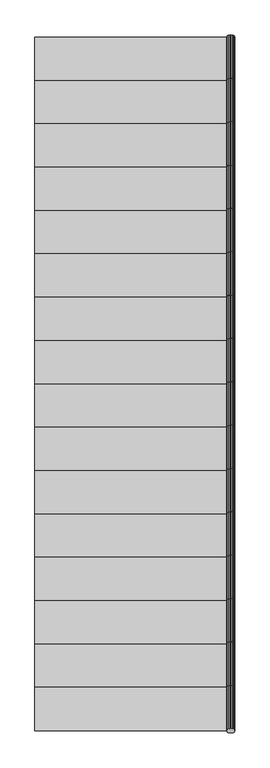
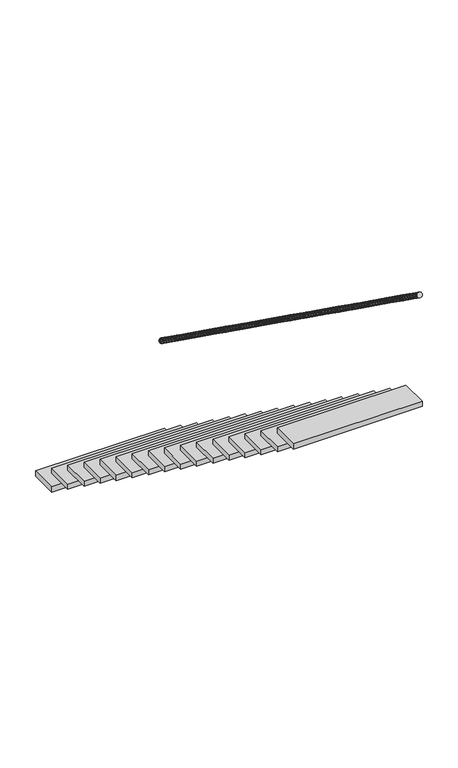
"""IFC4 building model written with IfcOpenShell, lengths in millimetres: stair geometry, 0_3d."""

from ifc_helpers import new_model, si_unit, frame, origin, origin_with_axes, place, context, project, spatial, polyline, outline, extrude, source, transform, mapped, element, save


def stair_45912ed6(model_context):
    return source(origin(), model_context, "Body", "SweptSolid", [
        extrude(outline(polyline([(1.2235871, -7.1914682), (0.0, 0.0), (1.2235871, 7.1914683), (4.7745751, 13.6789855), (10.3053687, 18.8275083), (17.2745751, 22.1330636), (25.0, 23.2720802), (32.7254249, 22.1330636), (39.6946313, 18.8275083), (45.2254249, 13.6789855), (48.7764129, 7.1914683), (50.0, 0.0), (48.7764129, -7.1914682), (45.2254249, -13.6789855), (39.6946313, -18.8275083), (32.7254249, -22.1330635), (25.0, -23.2720801), (17.2745751, -22.1330635), (10.3053687, -18.8275083), (4.7745751, -13.6789855), (1.2235871, -7.1914682)])), frame((1150.0, 3653.5347238, 1292.7647059), z_axis=(0.0, -0.8134846854822023, 0.5815863362269806), x_axis=(1.0, 0.0, 0.0)), (0.0, 0.0, 1.0), 319.6126548),
        extrude(outline(polyline([(1.2235871, -7.1914682), (0.0, 0.0), (1.2235871, 7.1914683), (4.7745751, 13.6789855), (10.3053687, 18.8275083), (17.2745751, 22.1330636), (25.0, 23.2720802), (32.7254249, 22.1330636), (39.6946313, 18.8275083), (45.2254249, 13.6789855), (48.7764129, 7.1914683), (50.0, 0.0), (48.7764129, -7.1914682), (45.2254249, -13.6789855), (39.6946313, -18.8275083), (32.7254249, -22.1330635), (25.0, -23.2720801), (17.2745751, -22.1330635), (10.3053687, -18.8275083), (4.7745751, -13.6789855), (1.2235871, -7.1914682)])), frame((1150.0, 4173.5347238, 921.0), z_axis=(0.0, -0.8134846854822141, 0.5815863362269641), x_axis=(1.0, 0.0, 0.0)), (0.0, 0.0, 1.0), 319.6126548),
        extrude(outline(polyline([(1.2235871, -7.1914682), (0.0, 0.0), (1.2235871, 7.1914683), (4.7745751, 13.6789855), (10.3053687, 18.8275083), (17.2745751, 22.1330636), (25.0, 23.2720802), (32.7254249, 22.1330636), (39.6946313, 18.8275083), (45.2254249, 13.6789855), (48.7764129, 7.1914683), (50.0, 0.0), (48.7764129, -7.1914682), (45.2254249, -13.6789855), (39.6946313, -18.8275083), (32.7254249, -22.1330635), (25.0, -23.2720801), (17.2745751, -22.1330635), (10.3053687, -18.8275083), (4.7745751, -13.6789855), (1.2235871, -7.1914682)])), frame((1150.0, 1833.5347238, 2593.9411765), z_axis=(0.0, -0.8134846854822316, 0.5815863362269396), x_axis=(1.0, 0.0, 0.0)), (0.0, 0.0, 1.0), 319.6126548),
        extrude(outline(polyline([(1.2235871, -7.1914682), (0.0, 0.0), (1.2235871, 7.1914683), (4.7745751, 13.6789855), (10.3053687, 18.8275083), (17.2745751, 22.1330636), (25.0, 23.2720802), (32.7254249, 22.1330636), (39.6946313, 18.8275083), (45.2254249, 13.6789855), (48.7764129, 7.1914683), (50.0, 0.0), (48.7764129, -7.1914682), (45.2254249, -13.6789855), (39.6946313, -18.8275083), (32.7254249, -22.1330635), (25.0, -23.2720801), (17.2745751, -22.1330635), (10.3053687, -18.8275083), (4.7745751, -13.6789855), (1.2235871, -7.1914682)])), frame((1150.0, 533.5347238, 3523.3529412), z_axis=(0.0, -0.8134846854822048, 0.581586336226977), x_axis=(1.0, 0.0, 0.0)), (0.0, 0.0, 1.0), 319.6126548),
        extrude(outline(polyline([(1.2235871, -7.1914682), (0.0, 0.0), (1.2235871, 7.1914683), (4.7745751, 13.6789855), (10.3053687, 18.8275083), (17.2745751, 22.1330636), (25.0, 23.2720802), (32.7254249, 22.1330636), (39.6946313, 18.8275083), (45.2254249, 13.6789855), (48.7764129, 7.1914683), (50.0, 0.0), (48.7764129, -7.1914682), (45.2254249, -13.6789855), (39.6946313, -18.8275083), (32.7254249, -22.1330635), (25.0, -23.2720801), (17.2745751, -22.1330635), (10.3053687, -18.8275083), (4.7745751, -13.6789855), (1.2235871, -7.1914682)])), frame((1150.0, 1053.5347238, 3151.5882353), z_axis=(0.0, -0.8134846854821998, 0.5815863362269841), x_axis=(1.0, 0.0, 0.0)), (0.0, 0.0, 1.0), 319.6126548),
        extrude(outline(polyline([(1.2235871, -7.1914682), (0.0, 0.0), (1.2235871, 7.1914683), (4.7745751, 13.6789855), (10.3053687, 18.8275083), (17.2745751, 22.1330636), (25.0, 23.2720802), (32.7254249, 22.1330636), (39.6946313, 18.8275083), (45.2254249, 13.6789855), (48.7764129, 7.1914683), (50.0, 0.0), (48.7764129, -7.1914682), (45.2254249, -13.6789855), (39.6946313, -18.8275083), (32.7254249, -22.1330635), (25.0, -23.2720801), (17.2745751, -22.1330635), (10.3053687, -18.8275083), (4.7745751, -13.6789855), (1.2235871, -7.1914682)])), frame((1150.0, 1573.5347238, 2779.8235294), z_axis=(0.0, -0.8134846854822146, 0.5815863362269632), x_axis=(1.0, 0.0, 0.0)), (0.0, 0.0, 1.0), 319.6126548),
        extrude(outline(polyline([(1200.0, 4173.5347238), (1200.0, 3913.5347238), (0.0, 3913.5347238), (0.0, 4173.5347238), (1200.0, 4173.5347238)])), origin_with_axes(), (0.0, 0.0, 1.0), 50.0),
        extrude(outline(polyline([(1.2235871, -7.1914682), (0.0, 0.0), (1.2235871, 7.1914683), (4.7745751, 13.6789856), (10.3053687, 18.8275083), (17.2745751, 22.1330636), (25.0, 23.2720803), (32.7254249, 22.1330636), (39.6946313, 18.8275083), (45.2254249, 13.6789856), (48.7764129, 7.1914683), (50.0, 0.0), (48.7764129, -7.1914682), (45.2254249, -13.6789855), (39.6946313, -18.8275083), (32.7254249, -22.1330635), (25.0, -23.2720801), (17.2745751, -22.1330635), (10.3053687, -18.8275083), (4.7745751, -13.6789855), (1.2235871, -7.1914682)])), frame((1150.0, 793.5347238, 3337.4705882), z_axis=(0.0, -0.8134846854821957, 0.5815863362269899), x_axis=(1.0, 0.0, 0.0)), (0.0, 0.0, 1.0), 319.6126548),
        extrude(outline(polyline([(1200.0, 2353.5347238), (1200.0, 2093.5347238), (0.0, 2093.5347238), (0.0, 2353.5347238), (1200.0, 2353.5347238)])), frame((0.0, 0.0, 1301.1764706), z_axis=(0.0, 0.0, 1.0), x_axis=(1.0, 0.0, 0.0)), (0.0, 0.0, 1.0), 50.0),
        extrude(outline(polyline([(1200.0, 3133.5347238), (1200.0, 2873.5347238), (0.0, 2873.5347238), (0.0, 3133.5347238), (1200.0, 3133.5347238)])), frame((0.0, 0.0, 743.5294118), z_axis=(0.0, 0.0, 1.0), x_axis=(1.0, 0.0, 0.0)), (0.0, 0.0, 1.0), 50.0),
        extrude(outline(polyline([(1.2235871, -7.1914682), (0.0, 0.0), (1.2235871, 7.1914683), (4.7745751, 13.6789855), (10.3053687, 18.8275083), (17.2745751, 22.1330636), (25.0, 23.2720802), (32.7254249, 22.1330636), (39.6946313, 18.8275083), (45.2254249, 13.6789855), (48.7764129, 7.1914683), (50.0, 0.0), (48.7764129, -7.1914682), (45.2254249, -13.6789855), (39.6946313, -18.8275083), (32.7254249, -22.1330635), (25.0, -23.2720801), (17.2745751, -22.1330635), (10.3053687, -18.8275083), (4.7745751, -13.6789855), (1.2235871, -7.1914682)])), frame((1150.0, 2353.5347238, 2222.1764706), z_axis=(0.0, -0.8134846854822106, 0.5815863362269689), x_axis=(1.0, 0.0, 0.0)), (0.0, 0.0, 1.0), 319.6126548),
        extrude(outline(polyline([(1.2235871, -7.1914682), (0.0, 0.0), (1.2235871, 7.1914683), (4.7745751, 13.6789855), (10.3053687, 18.8275083), (17.2745751, 22.1330636), (25.0, 23.2720802), (32.7254249, 22.1330636), (39.6946313, 18.8275083), (45.2254249, 13.6789855), (48.7764129, 7.1914683), (50.0, 0.0), (48.7764129, -7.1914682), (45.2254249, -13.6789855), (39.6946313, -18.8275083), (32.7254249, -22.1330635), (25.0, -23.2720801), (17.2745751, -22.1330635), (10.3053687, -18.8275083), (4.7745751, -13.6789855), (1.2235871, -7.1914682)])), frame((1150.0, 273.5347238, 3709.2352941), z_axis=(0.0, -0.8134846854821822, 0.5815863362270085), x_axis=(1.0, 0.0, 0.0)), (0.0, 0.0, 1.0), 319.6126548),
        extrude(outline(polyline([(1200.0, 1313.5347238), (1200.0, 1053.5347238), (0.0, 1053.5347238), (0.0, 1313.5347238), (1200.0, 1313.5347238)])), frame((0.0, 0.0, 2044.7058824), z_axis=(0.0, 0.0, 1.0), x_axis=(1.0, 0.0, 0.0)), (0.0, 0.0, 1.0), 50.0),
        extrude(outline(polyline([(1200.0, 3913.5347238), (1200.0, 3653.5347238), (0.0, 3653.5347238), (0.0, 3913.5347238), (1200.0, 3913.5347238)])), frame((0.0, 0.0, 185.8823529), z_axis=(0.0, 0.0, 1.0), x_axis=(1.0, 0.0, 0.0)), (0.0, 0.0, 1.0), 50.0),
        extrude(outline(polyline([(1200.0, 533.5347238), (1200.0, 273.5347238), (0.0, 273.5347238), (0.0, 533.5347238), (1200.0, 533.5347238)])), frame((0.0, 0.0, 2602.3529412), z_axis=(0.0, 0.0, 1.0), x_axis=(1.0, 0.0, 0.0)), (0.0, 0.0, 1.0), 50.0),
        extrude(outline(polyline([(1200.0, 2093.5347238), (1200.0, 1833.5347238), (0.0, 1833.5347238), (0.0, 2093.5347238), (1200.0, 2093.5347238)])), frame((0.0, 0.0, 1487.0588235), z_axis=(0.0, 0.0, 1.0), x_axis=(1.0, 0.0, 0.0)), (0.0, 0.0, 1.0), 50.0),
        extrude(outline(polyline([(1200.0, 1053.5347238), (1200.0, 793.5347238), (0.0, 793.5347238), (0.0, 1053.5347238), (1200.0, 1053.5347238)])), frame((0.0, 0.0, 2230.5882353), z_axis=(0.0, 0.0, 1.0), x_axis=(1.0, 0.0, 0.0)), (0.0, 0.0, 1.0), 50.0),
        extrude(outline(polyline([(1200.0, 3393.5347238), (1200.0, 3133.5347238), (0.0, 3133.5347238), (0.0, 3393.5347238), (1200.0, 3393.5347238)])), frame((0.0, 0.0, 557.6470588), z_axis=(0.0, 0.0, 1.0), x_axis=(1.0, 0.0, 0.0)), (0.0, 0.0, 1.0), 50.0),
        extrude(outline(polyline([(1.2235871, -7.1914682), (0.0, 0.0), (1.2235871, 7.1914683), (4.7745751, 13.6789855), (10.3053687, 18.8275083), (17.2745751, 22.1330636), (25.0, 23.2720802), (32.7254249, 22.1330636), (39.6946313, 18.8275083), (45.2254249, 13.6789855), (48.7764129, 7.1914683), (50.0, 0.0), (48.7764129, -7.1914682), (45.2254249, -13.6789855), (39.6946313, -18.8275083), (32.7254249, -22.1330635), (25.0, -23.2720801), (17.2745751, -22.1330635), (10.3053687, -18.8275083), (4.7745751, -13.6789855), (1.2235871, -7.1914682)])), frame((1150.0, 2873.5347238, 1850.4117647), z_axis=(0.0, -0.813484685482208, 0.5815863362269725), x_axis=(1.0, 0.0, 0.0)), (0.0, 0.0, 1.0), 319.6126548),
        extrude(outline(polyline([(1200.0, 793.5347238), (1200.0, 533.5347238), (0.0, 533.5347238), (0.0, 793.5347238), (1200.0, 793.5347238)])), frame((0.0, 0.0, 2416.4705882), z_axis=(0.0, 0.0, 1.0), x_axis=(1.0, 0.0, 0.0)), (0.0, 0.0, 1.0), 50.0),
        extrude(outline(polyline([(1200.0, 273.5347238), (1200.0, 13.5347238), (0.0, 13.5347238), (0.0, 273.5347238), (1200.0, 273.5347238)])), frame((0.0, 0.0, 2788.2352941), z_axis=(0.0, 0.0, 1.0), x_axis=(1.0, 0.0, 0.0)), (0.0, 0.0, 1.0), 50.0),
        extrude(outline(polyline([(1200.0, 2613.5347238), (1200.0, 2353.5347238), (0.0, 2353.5347238), (0.0, 2613.5347238), (1200.0, 2613.5347238)])), frame((0.0, 0.0, 1115.2941176), z_axis=(0.0, 0.0, 1.0), x_axis=(1.0, 0.0, 0.0)), (0.0, 0.0, 1.0), 50.0),
        extrude(outline(polyline([(1.2235871, -7.1914682), (0.0, 0.0), (1.2235871, 7.1914683), (4.7745751, 13.6789856), (10.3053687, 18.8275084), (17.2745751, 22.1330636), (25.0, 23.2720803), (32.7254249, 22.1330636), (39.6946313, 18.8275084), (45.2254249, 13.6789856), (48.7764129, 7.1914683), (50.0, 0.0), (48.7764129, -7.1914682), (45.2254249, -13.6789855), (39.6946313, -18.8275083), (32.7254249, -22.1330635), (25.0, -23.2720801), (17.2745751, -22.1330635), (10.3053687, -18.8275083), (4.7745751, -13.6789855), (1.2235871, -7.1914682)])), frame((1150.0, 3913.5347238, 1106.8823529), z_axis=(0.0, -0.8134846854822255, 0.5815863362269482), x_axis=(1.0, 0.0, 0.0)), (0.0, 0.0, 1.0), 319.6126548),
        extrude(outline(polyline([(1200.0, 3653.5347238), (1200.0, 3393.5347238), (0.0, 3393.5347238), (0.0, 3653.5347238), (1200.0, 3653.5347238)])), frame((0.0, 0.0, 371.7647059), z_axis=(0.0, 0.0, 1.0), x_axis=(1.0, 0.0, 0.0)), (0.0, 0.0, 1.0), 50.0),
        extrude(outline(polyline([(1.2235871, -7.1914682), (0.0, 0.0), (1.2235871, 7.1914683), (4.7745751, 13.6789856), (10.3053687, 18.8275083), (17.2745751, 22.1330636), (25.0, 23.2720802), (32.7254249, 22.1330636), (39.6946313, 18.8275083), (45.2254249, 13.6789856), (48.7764129, 7.1914683), (50.0, 0.0), (48.7764129, -7.1914682), (45.2254249, -13.6789855), (39.6946313, -18.8275083), (32.7254249, -22.1330635), (25.0, -23.2720801), (17.2745751, -22.1330635), (10.3053687, -18.8275083), (4.7745751, -13.6789855), (1.2235871, -7.1914682)])), frame((1150.0, 3393.5347238, 1478.6470588), z_axis=(0.0, -0.8134846854822252, 0.5815863362269487), x_axis=(1.0, 0.0, 0.0)), (0.0, 0.0, 1.0), 319.6126548),
        extrude(outline(polyline([(1200.0, 1573.5347238), (1200.0, 1313.5347238), (0.0, 1313.5347238), (0.0, 1573.5347238), (1200.0, 1573.5347238)])), frame((0.0, 0.0, 1858.8235294), z_axis=(0.0, 0.0, 1.0), x_axis=(1.0, 0.0, 0.0)), (0.0, 0.0, 1.0), 50.0),
        extrude(outline(polyline([(1200.0, 2873.5347238), (1200.0, 2613.5347238), (0.0, 2613.5347238), (0.0, 2873.5347238), (1200.0, 2873.5347238)])), frame((0.0, 0.0, 929.4117647), z_axis=(0.0, 0.0, 1.0), x_axis=(1.0, 0.0, 0.0)), (0.0, 0.0, 1.0), 50.0),
        extrude(outline(polyline([(1.2235871, -7.1914682), (0.0, 0.0), (1.2235871, 7.1914683), (4.7745751, 13.6789855), (10.3053687, 18.8275083), (17.2745751, 22.1330635), (25.0, 23.2720802), (32.7254249, 22.1330635), (39.6946313, 18.8275083), (45.2254249, 13.6789855), (48.7764129, 7.1914683), (50.0, 0.0), (48.7764129, -7.1914682), (45.2254249, -13.6789855), (39.6946313, -18.8275084), (32.7254249, -22.1330635), (25.0, -23.2720802), (17.2745751, -22.1330635), (10.3053687, -18.8275084), (4.7745751, -13.6789855), (1.2235871, -7.1914682)])), frame((1150.0, 1313.5347238, 2965.7058824), z_axis=(0.0, -0.81348468548223, 0.5815863362269419), x_axis=(1.0, 0.0, 0.0)), (0.0, 0.0, 1.0), 319.6126548),
        extrude(outline(polyline([(1.2235871, -7.1914682), (0.0, 0.0), (1.2235871, 7.1914683), (4.7745751, 13.6789856), (10.3053687, 18.8275083), (17.2745751, 22.1330636), (25.0, 23.2720802), (32.7254249, 22.1330636), (39.6946313, 18.8275083), (45.2254249, 13.6789856), (48.7764129, 7.1914683), (50.0, 0.0), (48.7764129, -7.1914682), (45.2254249, -13.6789855), (39.6946313, -18.8275083), (32.7254249, -22.1330635), (25.0, -23.2720801), (17.2745751, -22.1330635), (10.3053687, -18.8275083), (4.7745751, -13.6789855), (1.2235871, -7.1914682)])), frame((1150.0, 2093.5347238, 2408.0588235), z_axis=(0.0, -0.8134846854821992, 0.5815863362269849), x_axis=(1.0, 0.0, 0.0)), (0.0, 0.0, 1.0), 319.6126548),
        extrude(outline(polyline([(1200.0, 1833.5347238), (1200.0, 1573.5347238), (0.0, 1573.5347238), (0.0, 1833.5347238), (1200.0, 1833.5347238)])), frame((0.0, 0.0, 1672.9411765), z_axis=(0.0, 0.0, 1.0), x_axis=(1.0, 0.0, 0.0)), (0.0, 0.0, 1.0), 50.0),
        extrude(outline(polyline([(1.2235871, -7.1914682), (0.0, 0.0), (1.2235871, 7.1914683), (4.7745751, 13.6789856), (10.3053687, 18.8275084), (17.2745751, 22.1330636), (25.0, 23.2720803), (32.7254249, 22.1330636), (39.6946313, 18.8275084), (45.2254249, 13.6789856), (48.7764129, 7.1914683), (50.0, 0.0), (48.7764129, -7.1914682), (45.2254249, -13.6789855), (39.6946313, -18.8275083), (32.7254249, -22.1330634), (25.0, -23.2720801), (17.2745751, -22.1330634), (10.3053687, -18.8275083), (4.7745751, -13.6789855), (1.2235871, -7.1914682)])), frame((1150.0, 2613.5347238, 2036.2941176), z_axis=(0.0, -0.8134846854822039, 0.5815863362269784), x_axis=(1.0, 0.0, 0.0)), (0.0, 0.0, 1.0), 319.6126548),
        extrude(outline(polyline([(1.2235871, -7.1914682), (0.0, 0.0), (1.2235871, 7.1914683), (4.7745751, 13.6789855), (10.3053687, 18.8275083), (17.2745751, 22.1330636), (25.0, 23.2720802), (32.7254249, 22.1330636), (39.6946313, 18.8275083), (45.2254249, 13.6789855), (48.7764129, 7.1914683), (50.0, 0.0), (48.7764129, -7.1914682), (45.2254249, -13.6789855), (39.6946313, -18.8275083), (32.7254249, -22.1330635), (25.0, -23.2720802), (17.2745751, -22.1330635), (10.3053687, -18.8275083), (4.7745751, -13.6789855), (1.2235871, -7.1914682)])), frame((1150.0, 3133.5347238, 1664.5294118), z_axis=(0.0, -0.813484685482228, 0.5815863362269446), x_axis=(1.0, 0.0, 0.0)), (0.0, 0.0, 1.0), 319.6126548),
    ])


if __name__ == "__main__":
    model = new_model("IFC4")
    model_context = context("Model", 3, world=origin())
    ifc_project = project(units=[si_unit("LENGTHUNIT", "METRE", prefix="MILLI")], contexts=[model_context])
    site = spatial("IfcSite", under=ifc_project)
    building = spatial("IfcBuilding", under=site)
    placement = place(None, origin())
    stair_shape = stair_45912ed6(model_context)
    element("IfcStair", 1, ObjectType="0_3d", at=placement, inside=building, context=model_context, shape_type="MappedRepresentation", body=[
        mapped(stair_shape, transform((0.0, 0.0, 0.0), x_axis=(1.0, 0.0, 0.0), y_axis=(0.0, 1.0, 0.0), z_axis=(0.0, 0.0, 1.0))),
    ])
    save(model, "model.ifc")

# Revit data of these elements
# Element 1 (IfcStair, "0_3d")
#   Materials on its faces: "*1", "weiss"
# Materials
#   "*1": class "Unassigned", colour RGB 175 175 175, transparency 0
#   "weiss": class "Unassigned", colour RGB 255 255 255, transparency 0
